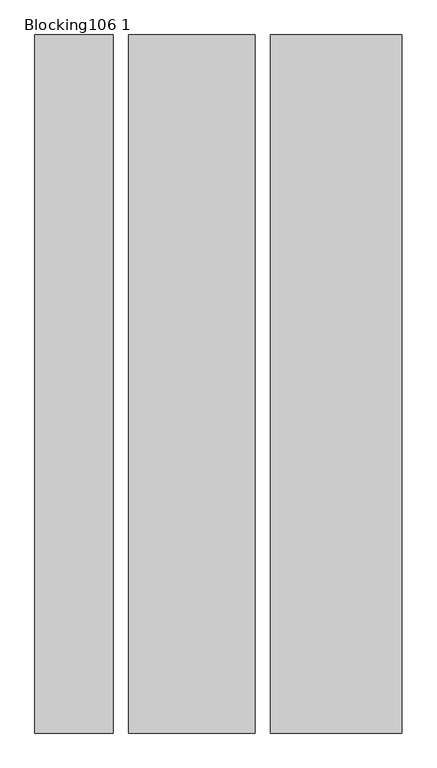
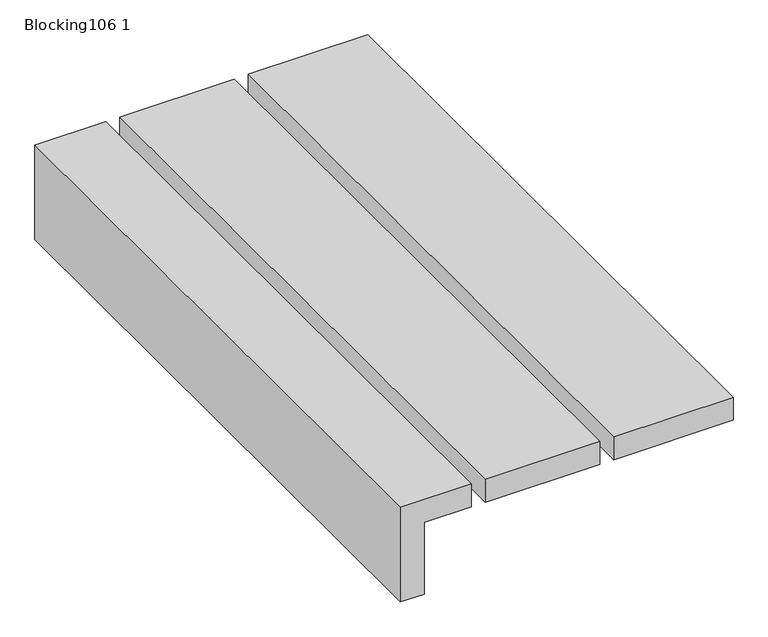
"""IFC4 building model written with IfcOpenShell, lengths in millimetres: proxy geometry, Blocking106 1 : Blocking106 12412."""

from ifc_helpers import new_model, si_unit, frame, origin, place, context, project, spatial, polyline, outline, extrude, source, transform, mapped, element, save


def blocking106_1_2ceb33a1(model_context):
    return source(origin(), model_context, "Body", "SweptSolid", [
        extrude(outline(polyline([(44042.7623529, 6172.6163563), (44042.7623529, 6320.6984495), (44118.9623529, 6320.6984495), (44118.9623529, 6096.4163563), (43803.0227817, 6096.4163563), (43803.0227817, 6172.6163563), (44042.7623529, 6172.6163563)])), frame((0.0, -1052.8908936, 0.0), z_axis=(0.0, 1.0, 0.0), x_axis=(0.0, 0.0, 1.0)), (0.0, 0.0, 1.0), 2000.0),
        extrude(outline(polyline([(7149.3612048, -1052.8908936), (6771.5484495, -1052.8908936), (6771.5484495, 947.1091064), (7149.3612048, 947.1091064), (7149.3612048, -1052.8908936)])), frame((0.0, 0.0, 44042.7623529), z_axis=(0.0, 0.0, 1.0), x_axis=(1.0, 0.0, 0.0)), (0.0, 0.0, 1.0), 76.2),
        extrude(outline(polyline([(6727.0984495, -1052.8908936), (6365.1484495, -1052.8908936), (6365.1484495, 947.1091064), (6727.0984495, 947.1091064), (6727.0984495, -1052.8908936)])), frame((0.0, 0.0, 44042.7623529), z_axis=(0.0, 0.0, 1.0), x_axis=(1.0, 0.0, 0.0)), (0.0, 0.0, 1.0), 76.2),
    ])


if __name__ == "__main__":
    model = new_model("IFC4")
    model_context = context("Model", 3, world=origin())
    ifc_project = project(units=[si_unit("LENGTHUNIT", "METRE", prefix="MILLI")], contexts=[model_context])
    site = spatial("IfcSite", under=ifc_project)
    building = spatial("IfcBuilding", under=site)
    placement = place(None, origin())
    blocking106_1_shape = blocking106_1_2ceb33a1(model_context)
    element("IfcBuildingElementProxy", 1, Name="Blocking106 1 : Blocking106 12412", ObjectType="Blocking106 1 : Blocking106 12412", at=placement, inside=building, context=model_context, shape_type="MappedRepresentation", body=[
        mapped(blocking106_1_shape, transform((0.0, 0.0, 0.0), x_axis=(1.0, 0.0, 0.0), y_axis=(0.0, 1.0, 0.0), z_axis=(0.0, 0.0, 1.0))),
    ])
    save(model, "model.ifc")

# Revit data of these elements
# Type "Blocking106 1 : Blocking106 12412"
#   NameOverride = "Blocking106"
# Element 1 (IfcBuildingElementProxy, "Blocking106 1 : Blocking106 12412")
#   Materials on its faces: "3\" POLYURETHANE SPRAY FOAM UNDER ROOF SUBSTRATE"
# Materials
#   "3\" POLYURETHANE SPRAY FOAM UNDER ROOF SUBSTRATE": class "Unassigned", colour RGB 210 164 194, transparency 0, Cost = 0
